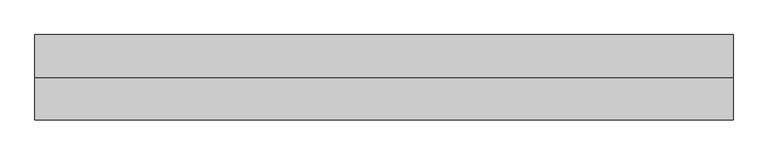
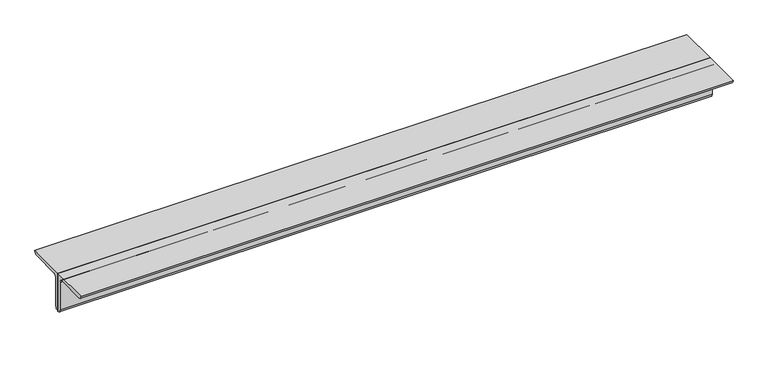
"""IFC4 building model written with IfcOpenShell, lengths in millimetres: beam geometry, 0123_Steel Framing_2Ls-KSD3502 : H_SB_AR_S04_2Ls-130x130x12_VBR1."""

from ifc_helpers import new_model, si_unit, point, frame, frame_2d, origin, place, context, project, spatial, polyline, circle_curve, trimmed, segment, composite_curve, outline, extrude, source, transform, mapped, element, save


def beam_a6789790(model_context):
    return source(origin(), model_context, "Body", "SweptSolid", [
        extrude(outline(composite_curve([segment(polyline([(0.0, 36.4), (130.0, 36.4)]), True, "CONTINUOUS"), segment(trimmed(circle_curve(frame_2d((118.0, 36.4)), 12.0), [point((130.0, 36.4))], [point((118.0, 24.4))], False, "CARTESIAN"), True, "CONTINUOUS"), segment(polyline([(118.0, 24.4), (24.0, 24.4)]), True, "CONTINUOUS"), segment(trimmed(circle_curve(frame_2d((24.0, 12.4)), 12.0), [point((24.0, 24.4))], [point((12.0, 12.4))], True, "CARTESIAN"), True, "CONTINUOUS"), segment(polyline([(12.0, 12.4), (12.0, -81.6)]), True, "CONTINUOUS"), segment(trimmed(circle_curve(frame_2d((0.0, -81.6)), 12.0), [point((12.0, -81.6))], [point((0.0, -93.6))], False, "CARTESIAN"), True, "CONTINUOUS"), segment(polyline([(0.0, -93.6), (0.0, 36.4)]), True, "CONTINUOUS")], self_intersect=False)), frame((-1023.6979116, 0.0, 0.0), z_axis=(1.0, 0.0, 0.0), x_axis=(0.0, 1.0, 0.0)), (0.0, 0.0, 1.0), 2122.0741046),
        extrude(outline(composite_curve([segment(polyline([(0.0, 36.4), (0.0, -93.6)]), True, "CONTINUOUS"), segment(trimmed(circle_curve(frame_2d((0.0, -81.6)), 12.0), [point((0.0, -93.6))], [point((-12.0, -81.6))], False, "CARTESIAN"), True, "CONTINUOUS"), segment(polyline([(-12.0, -81.6), (-12.0, 12.4)]), True, "CONTINUOUS"), segment(trimmed(circle_curve(frame_2d((-24.0, 12.4)), 12.0), [point((-12.0, 12.4))], [point((-24.0, 24.4))], True, "CARTESIAN"), True, "CONTINUOUS"), segment(polyline([(-24.0, 24.4), (-118.0, 24.4)]), True, "CONTINUOUS"), segment(trimmed(circle_curve(frame_2d((-118.0, 36.4)), 12.0), [point((-118.0, 24.4))], [point((-130.0, 36.4))], False, "CARTESIAN"), True, "CONTINUOUS"), segment(polyline([(-130.0, 36.4), (0.0, 36.4)]), True, "CONTINUOUS")], self_intersect=False)), frame((-1023.6979116, 0.0, 0.0), z_axis=(1.0, 0.0, 0.0), x_axis=(0.0, 1.0, 0.0)), (0.0, 0.0, 1.0), 2122.0741046),
    ])


if __name__ == "__main__":
    model = new_model("IFC4")
    model_context = context("Model", 3, world=origin())
    ifc_project = project(units=[si_unit("LENGTHUNIT", "METRE", prefix="MILLI")], contexts=[model_context])
    site = spatial("IfcSite", under=ifc_project)
    building = spatial("IfcBuilding", under=site)
    placement = place(None, origin())
    beam_shape = beam_a6789790(model_context)
    element("IfcBeam", 1, ObjectType="0123_Steel Framing_2Ls-KSD3502 : H_SB_AR_S04_2Ls-130x130x12_VBR1", at=placement, inside=building, context=model_context, shape_type="MappedRepresentation", body=[
        mapped(beam_shape, transform((0.0, 0.0, 0.0), x_axis=(1.0, 0.0, 0.0), y_axis=(0.0, 1.0, 0.0), z_axis=(0.0, 0.0, 1.0))),
    ])
    save(model, "model.ifc")

# Revit data of these elements
# Type "0123_Steel Framing_2Ls-KSD3502 : H_SB_AR_S04_2Ls-130x130x12_VBR1"
#   Type Mark = "VBR1"
#   Assembly Code = "B10"
#   Legs = "SLBB"
#   W = 8.97
#   Perimeter = 1.04 m²/m
#   Nominal Weight = 46.80 kgf/m
#   Length [instance default] = 1000 mm
#   Space = 0 mm
#   b = 130 mm
#   d = 130 mm
#   t = 12 mm
#   y = 36.4 mm
#   A = 0.005952 m²
#   Structural Material [instance default] = Steel ASTM A36
# Element 1 (IfcBeam, "0123_Steel Framing_2Ls-KSD3502 : H_SB_AR_S04_2Ls-130x130x12_VBR1")
#   Materials on its faces: "Steel ASTM A36"
# Materials
#   "Steel ASTM A36": class "Metal", colour RGB 199 199 199, transparency 0, Description = "Structural steel, ASTM A36 Grade B, mill finish", Cost = 0
